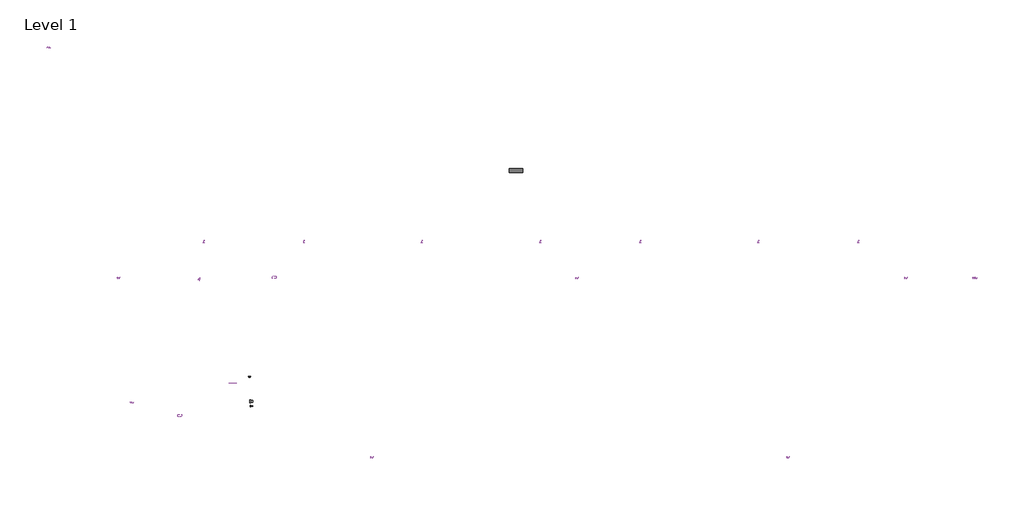
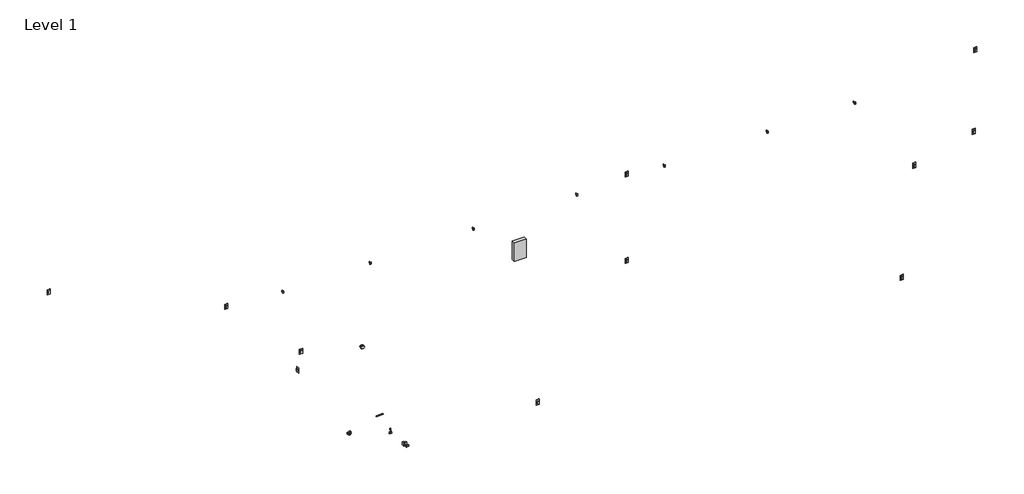
# One storey: 26 proxies.
# Revit data of these elements (continued)
# Type "Intruder Security Alarm Sounder : Standard" (continued)
#   Classification.MasterFormat.Number = "28 30 00"
#   Classification.OmniClass.23.Number = "23-29 11 23 15"
#   Classification.OmniClass.23.Description = "Intrusion Detection Microwave Alarms"
#   Classification.UniFormat.II.Number = "D7050"
#   COBie.Type.CreatedBy = "info@mma.ie"
#   COBie.Type.CreatedOn = "2017-07-26T09:25:07"
#   COBie.Type.Name = "Intruder Security Alarm Sounder"
#   COBie.Type.Category = "23-29 11 23 15 : Intrusion Detection Microwave Alarms"
#   COBie.Type.Description = "Intruder Security Alarm Sounder_Intruder Security Alarm Sounder"
#   COBie.Type.AssetType = "Fixed"
#   COBie.Type.Manufacturer = ""
#   COBie.Type.ModelNumber = ""
#   Standard = ""
#   SounderType = ""
#   SounderCutOffTimeMaximum = ""
#   PowerSupply = ""
#   Mounting = ""
#   Keynote = "28 01 30.51.A"
#   IntegralBeacon = ""
#   IngressProtectionStandard = ""
#   I.A. Audio Level = "75dB"
#   DirectionalOutputAt1MMinimum = ""
#   COBie.Type.ReplacementCost = 0
#   UsageCurrent = 0
#   SounderRadius = 75 mm
#   SounderDepth = 50 mm
#   PlanSymbolOffset [instance default] = 250 mm
#   PlanSymbolAlignment [instance default] = 0 mm
#   PhaseAngle = 0.00°
#   NominalVoltage = 0
#   NominalLength = 150 mm
#   NominalHeight = 80 mm
#   NominalFrequencyRange = 0
#   NominalCurrent = 0
#   I.A. Diameter = 150 mm
#   I.A. Depth = 50 mm
#   BaseLevelOffset = 0 mm
#   BackingCaseDepth = 30 mm
#   COBie.Type = yes
#   PlanSymbolVisibility [instance default] = yes
#   PlanObjectVisibility [instance default] = yes
#   NumberOfPoles = 0
#   HasProtectiveEarth = yes
#   URL = ""
#   Type Comments = ""
#   Model = ""
#   Manufacturer = ""
#   Description = (empty or 0)
#   Default Elevation = 0
#   Assembly Code = ""
# Type "Wall Mounted Passive Infrared Detector : Standard"
#   Type Mark = "Wall Mounted Passive Infrared Detector"
#   Classification.OmniClass.21.Number = "21-04 70 70 10"
#   Classification.OmniClass.21.Description = "Electronic Detention Monitoring and Control"
#   Classification.UniFormat.II.Description = "Intruction Detection"
#   Classification.OmniClass.23.Number = "23-29 11 21"
#   Classification.OmniClass.23.Description = "Security Sensors"
#   Classification.UniFormat.II.Number = "D7010.50"
#   COBie.Type.CreatedBy = "info@mma.ie"
#   COBie.Type.CreatedOn = "2017-07-26T09:12:44"
#   COBie.Type.Name = "Wall Mounted Passive Infrared Detector"
#   COBie.Type.Category = "23-29 11 21 : Security Sensors"
#   COBie.Type.Description = "Wall Mounted Passive Infrared Detector_Standard"
#   COBie.Type.AssetType = "Movable"
#   COBie.Type.Manufacturer = ""
#   COBie.Type.ModelNumber = ""
#   COBie.Type.ModelReference = ""
#   COBie.Type.Color = "White"
#   Units = "Volts"
#   Label = "PIR"
#   Keynote = "28 16 19.A"
#   COBie.Type.ReplacementCost = 0
#   Width 1 = 128 mm
#   Sensor Voltage = 230 V
#   PIR_Width = 64 mm
#   PIR_Depth = 53 mm
#   PIR Height = 117 mm
#   Length 1 = 234 mm
#   Height 1 = 3.312 mm
#   Default Elevation = 1200 mm
#   Sensor Width = 64 mm
#   Sensor Length = 117 mm
#   Sensor Height = 53 mm
#   Apparent Load = 0 VA
#   COBie.Type = yes
#   Sensor Number of Poles = 1
#   Sensor Material = none
#   Load Classification = Other
#   Cover Material = none
#   URL = ""
#   Model = ""
#   Manufacturer = ""
# Element 1 (IfcBuildingElementProxy, "Access Card Reader : Standard")
#   Comments = "2"
#   Mark = "1"
#   COBie.CreatedBy = "info@mma.ie"
#   COBie.CreatedOn = "2017-07-26T09:12:43"
#   COBie.Component.Name = "Access Card Reader-1"
#   COBie.Component.Space = "128"
#   COBie.Component.Description = "Access Card Reader: Standard"
#   Notes = "n/a"
#   Color = "Grey"
#   Voltage = 12 V
#   Power = 2.8 W
#   COBie = yes
#   Image = none
#   Phase Created = New Construction
# Element 2 (IfcBuildingElementProxy, "Access Card Reader : Standard")
#   Comments = "1"
#   Mark = "2"
#   COBie.CreatedBy = "info@mma.ie"
#   COBie.CreatedOn = "2017-07-26T09:12:43"
#   COBie.Component.Name = "Access Card Reader-2"
#   COBie.Component.Space = "217"
#   COBie.Component.Description = "Access Card Reader: Standard"
#   Notes = "n/a"
#   Color = "Grey"
#   Voltage = 12 V
#   Power = 2.8 W
#   COBie = yes
#   Phase Created = New Construction
# Element 3 (IfcBuildingElementProxy, "Access Card Reader : Standard")
#   Comments = "2"
#   Mark = "3"
#   COBie.CreatedBy = "info@mma.ie"
#   COBie.CreatedOn = "2017-07-26T09:12:43"
#   COBie.Component.Name = "Access Card Reader-3"
#   COBie.Component.Space = "217"
#   COBie.Component.Description = "Access Card Reader: Standard"
#   Notes = "n/a"
#   Color = "Grey"
#   Voltage = 12 V
#   Power = 2.8 W
#   COBie = yes
#   Phase Created = New Construction
# Element 4 (IfcBuildingElementProxy, "Access Card Reader : Standard")
#   Comments = "3"
#   Mark = "4"
#   COBie.CreatedBy = "info@mma.ie"
#   COBie.CreatedOn = "2017-07-26T09:12:43"
#   COBie.Component.Name = "Access Card Reader-4"
#   COBie.Component.Space = "217"
#   COBie.Component.Description = "Access Card Reader: Standard"
#   Notes = "n/a"
#   Color = "Grey"
#   Voltage = 12 V
#   Power = 2.8 W
#   COBie = yes
#   Phase Created = New Construction
# Element 5 (IfcBuildingElementProxy, "Access Card Reader : Standard")
#   Comments = "4"
#   Mark = "5"
#   COBie.CreatedBy = "info@mma.ie"
#   COBie.CreatedOn = "2017-07-26T09:12:43"
#   COBie.Component.Name = "Access Card Reader-5"
#   COBie.Component.Space = "217"
#   COBie.Component.Description = "Access Card Reader: Standard"
#   Notes = "n/a"
#   Color = "Grey"
#   Voltage = 12 V
#   Power = 2.8 W
#   COBie = yes
#   Phase Created = New Construction
# Element 6 (IfcBuildingElementProxy, "Access Card Reader : Standard")
#   Comments = "5"
#   Mark = "6"
#   COBie.CreatedBy = "info@mma.ie"
#   COBie.CreatedOn = "2017-07-26T09:12:43"
#   COBie.Component.Name = "Access Card Reader-6"
#   COBie.Component.Space = "217"
#   COBie.Component.Description = "Access Card Reader: Standard"
#   Notes = "n/a"
#   Color = "Grey"
#   Voltage = 12 V
#   Power = 2.8 W
#   COBie = yes
#   Phase Created = New Construction
# Element 7 (IfcBuildingElementProxy, "Access Card Reader : Standard")
#   Comments = "6"
#   Mark = "7"
#   COBie.CreatedBy = "info@mma.ie"
#   COBie.CreatedOn = "2017-07-26T09:12:43"
#   COBie.Component.Name = "Access Card Reader-7"
#   COBie.Component.Space = "217"
#   COBie.Component.Description = "Access Card Reader: Standard"
#   Notes = "n/a"
#   Color = "Grey"
#   Voltage = 12 V
#   Power = 2.8 W
#   COBie = yes
#   Phase Created = New Construction
# Element 8 (IfcBuildingElementProxy, "Access Card Reader : Standard")
#   Comments = "7"
#   Mark = "8"
#   COBie.CreatedBy = "info@mma.ie"
#   COBie.CreatedOn = "2017-07-26T09:12:43"
#   COBie.Component.Name = "Access Card Reader-8"
#   COBie.Component.Space = "217"
#   COBie.Component.Description = "Access Card Reader: Standard"
#   Notes = "n/a"
#   Color = "Grey"
#   Voltage = 12 V
#   Power = 2.8 W
#   COBie = yes
#   Phase Created = New Construction
# Element 9 (IfcBuildingElementProxy, "Bell : Standard")
#   Comments = "1"
#   Mark = "1"
#   COBie.CreatedBy = "info@mma.ie"
#   COBie.CreatedOn = "2017-07-26T09:12:43"
#   COBie.Component.Name = "Bell-1"
#   COBie.Component.Space = "128"
#   COBie.Component.Description = "Bell: Standard"
#   Notes = "n/a"
#   Color = "Silver"
#   Voltage = 12 V
#   Power = 2.8 W
#   COBie = yes
#   Phase Created = New Construction
# Element 10 (IfcBuildingElementProxy, "Door Lock Magnetic : Standard")
#   Comments = "14"
#   Mark = "1"
#   COBie.CreatedBy = "info@mma.ie"
#   COBie.CreatedOn = "2017-07-26T09:12:43"
#   COBie.Component.Name = "Door Lock Magnetic-1"
#   COBie.Component.Space = "123"
#   COBie.Component.Description = "Door Lock Magnetic: Standard"
#   Notes = "n/a"
#   Color = "Stainless Steel"
#   Voltage = 12 V
#   Power = 2.8 W
#   COBie = yes
#   Phase Created = New Construction
# Element 11 (IfcBuildingElementProxy, "Keypad : Standard")
#   Mark = "1"
#   COBie.CreatedBy = "info@mma.ie"
#   COBie.CreatedOn = "2017-07-26T09:12:43"
#   COBie.Component.Name = "Keypad-1"
#   COBie.Component.Space = "123"
#   COBie.Component.Description = "Keypad: Standard"
#   Notes = "n/a"
#   Color = "Stainless Steel"
#   Voltage = 12 V
#   Power = 3 W
#   COBie = yes
#   Phase Created = New Construction
# Element 12 (IfcBuildingElementProxy, "Release Button : Standard")
#   Comments = "5"
#   Mark = "1"
#   COBie.CreatedBy = "info@mma.ie"
#   COBie.CreatedOn = "2017-07-26T09:12:43"
#   COBie.Component.Name = "Release Button-1"
#   COBie.Component.Space = "123"
#   COBie.Component.Description = "Release Button: Standard"
#   Notes = "n/a"
#   Color = "Stainless Steel"
#   Voltage = 24 V
#   Power = 2.8 W
#   COBie = yes
#   Phase Created = New Construction
# Element 13 (IfcBuildingElementProxy, "Security Panel : 225 A")
#   Panel Name = "SP1"
#   Mark = "1"
#   COBie.CreatedBy = "info@mma.ie"
#   COBie.CreatedOn = "2017-07-26T09:12:43"
#   COBie.Component.Name = "Security Panel-1"
#   COBie.Component.Space = "107"
#   COBie.Component.Description = "Security Panel: 225 A"
#   Notes = "n/a"
#   Color = "Black"
#   built-in parameter 1140081 = "Recessed"
#   built-in parameter 1140083 = "Type 1"
#   Voltage = 208 V
#   built-in parameter 1140082 = 100 (stored number, unit not read)
#   Height = 812.8 mm
#   COBie = yes
#   built-in parameter 1140079 = 18
#   built-in parameter 1140064 = 120/208 Wye
#   Phase Created = New Construction
# Element 14 (IfcBuildingElementProxy, "Intruder Security Alarm Sounder : Standard")
#   Mark = "1"
#   COBie.CreatedBy = "info@mma.ie"
#   COBie.CreatedOn = "2017-07-26T09:12:43"
#   COBie.Component.Name = "Intruder Security Alarm Sounder-1"
#   COBie.Component.Space = "117"
#   COBie.Component.Description = "Intruder Security Alarm Sounder: Intruder Security Alarm Sounder"
#   Notes = "n/a"
#   Color = "Red"
#   Voltage = 24 V
#   Power = 0.6 W
#   PlanSymbolOffset = 250 mm
#   PlanSymbolAlignment = 0 mm
#   COBie = yes
#   PlanSymbolVisibility = yes
#   PlanObjectVisibility = yes
#   Phase Created = New Construction
#   Materials on its faces: "nbl_ConceptWhite"
# Element 15 (IfcBuildingElementProxy, "Intruder Security Alarm Sounder : Standard")
#   Mark = "2"
#   COBie.CreatedBy = "info@mma.ie"
#   COBie.CreatedOn = "2017-07-26T09:12:43"
#   COBie.Component.Name = "Intruder Security Alarm Sounder-2"
#   COBie.Component.Space = "128"
#   COBie.Component.Description = "Intruder Security Alarm Sounder: Intruder Security Alarm Sounder"
#   Notes = "n/a"
#   Color = "Red"
#   Voltage = 24 V
#   Power = 0.6 W
#   PlanSymbolOffset = 250 mm
#   PlanSymbolAlignment = 0 mm
#   COBie = yes
#   PlanSymbolVisibility = yes
#   PlanObjectVisibility = yes
#   Phase Created = New Construction
#   Materials on its faces: "nbl_ConceptWhite"
# Element 16 (IfcBuildingElementProxy, "Wall Mounted Passive Infrared Detector : Standard")
#   Comments = "6"
#   Mark = "1"
#   COBie.CreatedBy = "info@mma.ie"
#   COBie.CreatedOn = "2017-07-26T09:12:43"
#   COBie.Component.Name = "Wall Mounted Passive Infrared Detector-1"
#   COBie.Component.Space = "117"
#   COBie.Component.Description = "Wall Mounted Passive Infrared Detector: Standard"
#   Notes = "n/a"
#   Color = "White"
#   Voltage = 12 V
#   Power = 0.15 W
#   COBie = yes
#   Phase Created = New Construction
# Element 17 (IfcBuildingElementProxy, "Wall Mounted Passive Infrared Detector : Standard")
#   Comments = "8"
#   Mark = "2"
#   COBie.CreatedBy = "info@mma.ie"
#   COBie.CreatedOn = "2017-07-26T09:12:43"
#   COBie.Component.Name = "Wall Mounted Passive Infrared Detector-2"
#   COBie.Component.Space = "101"
#   COBie.Component.Description = "Wall Mounted Passive Infrared Detector: Standard"
#   Notes = "n/a"
#   Color = "White"
#   Voltage = 12 V
#   Power = 0.15 W
#   COBie = yes
#   Phase Created = New Construction
# Element 18 (IfcBuildingElementProxy, "Wall Mounted Passive Infrared Detector : Standard")
#   Comments = "9"
#   Mark = "3"
#   COBie.CreatedBy = "info@mma.ie"
#   COBie.CreatedOn = "2017-07-26T09:12:43"
#   COBie.Component.Name = "Wall Mounted Passive Infrared Detector-3"
#   COBie.Component.Space = "118"
#   COBie.Component.Description = "Wall Mounted Passive Infrared Detector: Standard"
#   Notes = "n/a"
#   Color = "White"
#   Voltage = 12 V
#   Power = 0.15 W
#   COBie = yes
#   Phase Created = New Construction
# Element 19 (IfcBuildingElementProxy, "Wall Mounted Passive Infrared Detector : Standard")
#   Comments = "8"
#   Mark = "4"
#   COBie.CreatedBy = "info@mma.ie"
#   COBie.CreatedOn = "2017-07-26T09:12:43"
#   COBie.Component.Name = "Wall Mounted Passive Infrared Detector-4"
#   COBie.Component.Space = "217"
#   COBie.Component.Description = "Wall Mounted Passive Infrared Detector: Standard"
#   Notes = "n/a"
#   Color = "White"
#   Voltage = 12 V
#   Power = 0.15 W
#   COBie = yes
#   Phase Created = New Construction
# Element 20 (IfcBuildingElementProxy, "Wall Mounted Passive Infrared Detector : Standard")
#   Comments = "10"
#   Mark = "6"
#   COBie.CreatedBy = "info@mma.ie"
#   COBie.CreatedOn = "2017-07-26T09:12:43"
#   COBie.Component.Name = "Wall Mounted Passive Infrared Detector-6"
#   COBie.Component.Space = "217"
#   COBie.Component.Description = "Wall Mounted Passive Infrared Detector: Standard"
#   Notes = "n/a"
#   Color = "White"
#   Voltage = 12 V
#   Power = 0.15 W
#   COBie = yes
#   Phase Created = New Construction
# Element 21 (IfcBuildingElementProxy, "Wall Mounted Passive Infrared Detector : Standard")
#   Comments = "12"
#   Mark = "7"
#   COBie.CreatedBy = "info@mma.ie"
#   COBie.CreatedOn = "2017-07-26T09:12:43"
#   COBie.Component.Name = "Wall Mounted Passive Infrared Detector-7"
#   COBie.Component.Space = "116"
#   COBie.Component.Description = "Wall Mounted Passive Infrared Detector: Standard"
#   Notes = "n/a"
#   Color = "White"
#   Voltage = 12 V
#   Power = 0.15 W
#   COBie = yes
#   Phase Created = New Construction
# Element 22 (IfcBuildingElementProxy, "Wall Mounted Passive Infrared Detector : Standard")
#   Comments = "11"
#   Mark = "8"
#   COBie.CreatedBy = "info@mma.ie"
#   COBie.CreatedOn = "2017-07-26T09:12:43"
#   COBie.Component.Name = "Wall Mounted Passive Infrared Detector-8"
#   COBie.Component.Space = "219"
#   COBie.Component.Description = "Wall Mounted Passive Infrared Detector: Standard"
#   Notes = "n/a"
#   Color = "White"
#   Voltage = 12 V
#   Power = 0.15 W
#   COBie = yes
#   Phase Created = New Construction
# Element 23 (IfcBuildingElementProxy, "Wall Mounted Passive Infrared Detector : Standard")
#   Comments = "12"
#   Mark = "9"
#   COBie.CreatedBy = "info@mma.ie"
#   COBie.CreatedOn = "2017-07-26T09:12:43"
#   COBie.Component.Name = "Wall Mounted Passive Infrared Detector-9"
#   COBie.Component.Space = "218"
#   COBie.Component.Description = "Wall Mounted Passive Infrared Detector: Standard"
#   Notes = "n/a"
#   Color = "White"
#   Voltage = 12 V
#   Power = 0.15 W
#   COBie = yes
#   Phase Created = New Construction
# Element 24 (IfcBuildingElementProxy, "Wall Mounted Passive Infrared Detector : Standard")
#   Comments = "16"
#   Mark = "10"
#   COBie.CreatedBy = "info@mma.ie"
#   COBie.CreatedOn = "2017-07-26T09:12:43"
#   COBie.Component.Name = "Wall Mounted Passive Infrared Detector-10"
#   COBie.Component.Space = "117"
#   COBie.Component.Description = "Wall Mounted Passive Infrared Detector: Standard"
#   Notes = "n/a"
#   Color = "White"
#   Voltage = 12 V
#   Power = 0.15 W
#   COBie = yes
#   Phase Created = New Construction
# Element 25 (IfcBuildingElementProxy, "Wall Mounted Passive Infrared Detector : Standard")
#   Comments = "17"
#   Mark = "11"
#   COBie.CreatedBy = "info@mma.ie"
#   COBie.CreatedOn = "2017-07-26T09:12:43"
#   COBie.Component.Name = "Wall Mounted Passive Infrared Detector-11"
#   COBie.Component.Space = "123"
#   COBie.Component.Description = "Wall Mounted Passive Infrared Detector: Standard"
#   Notes = "n/a"
#   Color = "White"
#   Voltage = 12 V
#   Power = 0.15 W
#   COBie = yes
#   Phase Created = New Construction
# Element 26 (IfcBuildingElementProxy, "Wall Mounted Passive Infrared Detector : Standard")
#   Comments = "9"
#   Mark = "12"
#   COBie.CreatedBy = "info@mma.ie"
#   COBie.CreatedOn = "2017-07-26T09:12:43"
#   COBie.Component.Name = "Wall Mounted Passive Infrared Detector-12"
#   COBie.Component.Space = "121"
#   COBie.Component.Description = "Wall Mounted Passive Infrared Detector: Standard"
#   Notes = "n/a"
#   Color = "White"
#   Voltage = 12 V
#   Power = 0.15 W
#   COBie = yes
#   Phase Created = New Construction
# Materials
#   "nbl_ConceptWhite": class "Generic", colour RGB 255 255 255, transparency 0, Cost = 0
# Space at (25106.444, 9340) mm, phase "New Construction", upper level "Level 2", upper offset -200 mm, lower offset 0 mm
#   Number = "111"
#   Name = "Storage"
#   Classification.Space.Number = "13-63 13 11"
#   Classification.Space.Description = "Storage Room"
#   COBie.CreatedBy = "info@mma.ie"
#   COBie.CreatedOn = "2017-07-26T09:12:43"
#   COBie.Space.Name = "111"
#   COBie.Space.Category = "13-63 13 11 : Storage Room"
#   COBie.Space.Description = "Storage"
#   Actual Lighting Load per area = 0
#   Actual Power Load per area = 0
#   Sensible Heat Gain per person = 0
#   Specified Lighting Load = 73041.7 (stored number, unit not read)
#   Specified Power Load = 94954.2 (stored number, unit not read)
#   Latent Heat Gain per person = 0
#   Total Heat Gain per person = 0
#   Area per Person = 0
#   Number of People = 22.0647 (stored number, unit not read)
#   COBie.Space.UsableHeight = 3600 mm
#   COBie.Space.GrossArea = 5.21302 m²
#   COBie.Space.NetArea = 0 m²
#   Lighting Load Units = 0
#   Power Load Units = 0
#   Return Airflow = 0
#   Occupancy Unit = -1
#   Condition Type = 2
#   COBie = yes
#   Construction Type = none
# Space at (-3466.111, 10795.59) mm, phase "New Construction", upper level "Level 2", upper offset 0 mm, lower offset 0 mm
#   Number = "001"
#   Name = "Exercise Terrace"
#   Classification.Space.Number = "13-33 11 15 41"
#   Classification.Space.Description = "Exercise Space"
#   COBie.CreatedBy = "info@mma.ie"
#   COBie.CreatedOn = "2017-07-26T09:12:43"
#   COBie.Space.Name = "001"
#   COBie.Space.Category = "13-33 11 15 41 : Exercise Space"
#   COBie.Space.Description = "Exercise Terrace"
#   Actual Lighting Load per area = 0
#   Actual Power Load per area = 0
#   Sensible Heat Gain per person = 0
#   Specified Lighting Load = 5865.96 (stored number, unit not read)
#   Specified Power Load = 7625.74 (stored number, unit not read)
#   Latent Heat Gain per person = 0
#   Total Heat Gain per person = 0
#   Area per Person = 0
#   Number of People = 1.77201 (stored number, unit not read)
#   COBie.Space.UsableHeight = 3800 mm
#   COBie.Space.GrossArea = 46.8469 m²
#   COBie.Space.NetArea = 0 m²
#   Lighting Load Units = 0
#   Power Load Units = 0
#   Return Airflow = 0
#   Occupancy Unit = -1
#   Condition Type = 2
#   COBie = yes
#   Construction Type = none
# Space at (6778.21, 4377.979) mm, phase "New Construction", upper level "Level 2", upper offset -200 mm, lower offset 0 mm
#   Number = "123"
#   Name = "Entry"
#   Classification.Space.Number = "13-25"
#   Classification.Space.Description = "Circulation Spaces"
#   COBie.CreatedBy = "info@mma.ie"
#   COBie.CreatedOn = "2017-07-26T09:12:43"
#   COBie.Space.Name = "123"
#   COBie.Space.Category = "13-25 : Circulation Spaces"
#   COBie.Space.Description = "Entry"
#   Actual Lighting Load per area = 0
#   Actual Power Load per area = 0
#   Sensible Heat Gain per person = 0
#   Specified Lighting Load = 1051.01 (stored number, unit not read)
#   Specified Power Load = 1366.31 (stored number, unit not read)
#   Latent Heat Gain per person = 0
#   Total Heat Gain per person = 0
#   Area per Person = 0
#   Number of People = 0.317492 (stored number, unit not read)
#   COBie.Space.UsableHeight = 3600 mm
#   COBie.Space.GrossArea = 7.40986 m²
#   COBie.Space.NetArea = 0 m²
#   Lighting Load Units = 0
#   Power Load Units = 0
#   Return Airflow = 0
#   Occupancy Unit = -1
#   Condition Type = 2
#   COBie = yes
#   Construction Type = none
# Space at (6131.224, -2983.196) mm, phase "New Construction", upper level "Level 1", upper offset 2000 mm, lower offset 0 mm
#   Number = "128"
#   Name = "External Space Level 1"
#   Classification.Space.Number = "13-25 17"
#   Classification.Space.Description = "External Circulation Spaces"
#   COBie.CreatedBy = "info@mma.ie"
#   COBie.CreatedOn = "2017-07-26T09:12:43"
#   COBie.Space.Name = "128"
#   COBie.Space.Category = "13-25 17 : External Circulation Spaces"
#   COBie.Space.Description = "External Circulation Spaces"
#   Actual Lighting Load per area = 0
#   Actual Power Load per area = 0
#   Sensible Heat Gain per person = 0
#   Specified Lighting Load = 80587.6 (stored number, unit not read)
#   Specified Power Load = 104763.9 (stored number, unit not read)
#   Latent Heat Gain per person = 0
#   Total Heat Gain per person = 0
#   Area per Person = 0
#   Number of People = 24.3442 (stored number, unit not read)
#   COBie.Space.UsableHeight = 2000 mm
#   COBie.Space.GrossArea = 695.172 m²
#   COBie.Space.NetArea = 0 m²
#   Lighting Load Units = 0
#   Power Load Units = 0
#   Return Airflow = 0
#   Occupancy Unit = -1
#   Condition Type = 2
#   COBie = yes
#   Construction Type = none
# Space at (30095.163, 9340) mm, phase "New Construction", upper level "Level 2", upper offset -200 mm, lower offset 0 mm
#   Number = "114"
#   Name = "Pantry"
#   Classification.Space.Number = "13-57 13 13"
#   Classification.Space.Description = "Kitchen Space"
#   COBie.CreatedBy = "info@mma.ie"
#   COBie.CreatedOn = "2017-07-26T09:12:43"
#   COBie.Space.Name = "114"
#   COBie.Space.Category = "13-57 13 13 : Kitchen Space"
#   COBie.Space.Description = "Pantry"
#   Actual Lighting Load per area = 0
#   Actual Power Load per area = 0
#   Sensible Heat Gain per person = 0
#   Specified Lighting Load = 0
#   Specified Power Load = 0
#   Latent Heat Gain per person = 0
#   Total Heat Gain per person = 0
#   Area per Person = 0
#   Number of People = 0.339922 (stored number, unit not read)
#   COBie.Space.UsableHeight = 3600 mm
#   COBie.Space.GrossArea = 9.71206 m²
#   COBie.Space.NetArea = 0 m²
#   Lighting Load Units = 0
#   Power Load Units = 0
#   Return Airflow = 0
#   Occupancy Unit = -1
#   Condition Type = 2
#   COBie = yes
#   Construction Type = none
# Space at (13314.806, 9198.95) mm, phase "New Construction", upper level "Level 2", upper offset -200 mm, lower offset 0 mm
#   Number = "104"
#   Name = "Storage"
#   Classification.Space.Number = "13-63 13 11"
#   Classification.Space.Description = "Storage Room"
#   COBie.CreatedBy = "info@mma.ie"
#   COBie.CreatedOn = "2017-07-26T09:12:43"
#   COBie.Space.Name = "104"
#   COBie.Space.Category = "13-63 13 11 : Storage Room"
#   COBie.Space.Description = "Storage"
#   Actual Lighting Load per area = 0
#   Actual Power Load per area = 0
#   Sensible Heat Gain per person = 0
#   Specified Lighting Load = 0
#   Specified Power Load = 0
#   Latent Heat Gain per person = 0
#   Total Heat Gain per person = 0
#   Area per Person = 0
#   Number of People = 0.36309 (stored number, unit not read)
#   COBie.Space.UsableHeight = 3600 mm
#   COBie.Space.GrossArea = 10.374 m²
#   COBie.Space.NetArea = 0 m²
#   Lighting Load Units = 0
#   Power Load Units = 0
#   Return Airflow = 0
#   Occupancy Unit = -1
#   Condition Type = 2
#   COBie = yes
#   Construction Type = none
# Space at (17230.963, 11648.082) mm, phase "New Construction", upper level "Level 2", upper offset -200 mm, lower offset 0 mm
#   Number = "107"
#   Name = "Closet"
#   Classification.Space.Number = "13-63 13 13"
#   Classification.Space.Description = "Closet"
#   COBie.CreatedBy = "info@mma.ie"
#   COBie.CreatedOn = "2017-07-26T09:12:43"
#   COBie.Space.Name = "107"
#   COBie.Space.Category = "13-63 13 13 : Closet"
#   COBie.Space.Description = "Closet"
#   Actual Lighting Load per area = 0
#   Actual Power Load per area = 0
#   Sensible Heat Gain per person = 0
#   Specified Lighting Load = 0
#   Specified Power Load = 0
#   Latent Heat Gain per person = 0
#   Total Heat Gain per person = 0
#   Area per Person = 0
#   Number of People = 0.0932222 (stored number, unit not read)
#   COBie.Space.UsableHeight = 3600 mm
#   COBie.Space.GrossArea = 2.66349 m²
#   COBie.Space.NetArea = 0 m²
#   Lighting Load Units = 0
#   Power Load Units = 0
#   Return Airflow = 0
#   Occupancy Unit = -1
#   Condition Type = 2
#   COBie = yes
#   Construction Type = none
# Space at (17230.963, 9449.188) mm, phase "New Construction", upper level "Level 2", upper offset -200 mm, lower offset 0 mm
#   Number = "109"
#   Name = "Elec/Tel"
#   Classification.Space.Number = "13-23 19 27"
#   Classification.Space.Description = "Electrical Room"
#   COBie.CreatedBy = "info@mma.ie"
#   COBie.CreatedOn = "2017-07-26T09:12:43"
#   COBie.Space.Name = "109"
#   COBie.Space.Category = "13-23 19 27 : Electrical Room"
#   COBie.Space.Description = "Elec/Tel"
#   Actual Lighting Load per area = 0
#   Actual Power Load per area = 0
#   Sensible Heat Gain per person = 0
#   Specified Lighting Load = 0
#   Specified Power Load = 0
#   Latent Heat Gain per person = 0
#   Total Heat Gain per person = 0
#   Area per Person = 0
#   Number of People = 0.141204 (stored number, unit not read)
#   COBie.Space.UsableHeight = 3600 mm
#   COBie.Space.GrossArea = 4.03441 m²
#   COBie.Space.NetArea = 0 m²
#   Lighting Load Units = 0
#   Power Load Units = 0
#   Return Airflow = 0
#   Occupancy Unit = -1
#   Condition Type = 2
#   COBie = yes
#   Construction Type = none
# Space at (20994.025, 9449.188) mm, phase "New Construction", upper level "Level 2", upper offset -200 mm, lower offset 0 mm
#   Number = "110"
#   Name = "Laundry"
#   Classification.Space.Number = "13-65 17"
#   Classification.Space.Description = "Laundry Room"
#   COBie.CreatedBy = "info@mma.ie"
#   COBie.CreatedOn = "2017-07-26T09:12:43"
#   COBie.Space.Name = "110"
#   COBie.Space.Category = "13-65 17 : Laundry Room"
#   COBie.Space.Description = "Laundry"
#   Actual Lighting Load per area = 0
#   Actual Power Load per area = 0
#   Sensible Heat Gain per person = 0
#   Specified Lighting Load = 0
#   Specified Power Load = 0
#   Latent Heat Gain per person = 0
#   Total Heat Gain per person = 0
#   Area per Person = 0
#   Number of People = 0.437432 (stored number, unit not read)
#   COBie.Space.UsableHeight = 3600 mm
#   COBie.Space.GrossArea = 12.4981 m²
#   COBie.Space.NetArea = 0 m²
#   Lighting Load Units = 0
#   Power Load Units = 0
#   Return Airflow = 0
#   Occupancy Unit = -1
#   Condition Type = 2
#   COBie = yes
#   Construction Type = none
# Space at (9483.263, 9198.95) mm, phase "New Construction", upper level "Level 2", upper offset -200 mm, lower offset 0 mm
#   Number = "103"
#   Name = "Toilet"
#   Classification.Space.Number = "13-65 13 13"
#   Classification.Space.Description = "Toilet Space"
#   COBie.CreatedBy = "info@mma.ie"
#   COBie.CreatedOn = "2017-07-26T09:12:43"
#   COBie.Space.Name = "103"
#   COBie.Space.Category = "13-65 13 13 : Toilet Space"
#   COBie.Space.Description = "Toilet"
#   Actual Lighting Load per area = 0
#   Actual Power Load per area = 0
#   Sensible Heat Gain per person = 0
#   Specified Lighting Load = 0
#   Specified Power Load = 0
#   Latent Heat Gain per person = 0
#   Total Heat Gain per person = 0
#   Area per Person = 0
#   Number of People = 0.146893 (stored number, unit not read)
#   COBie.Space.UsableHeight = 3600 mm
#   COBie.Space.GrossArea = 4.19694 m²
#   COBie.Space.NetArea = 0 m²
#   Lighting Load Units = 0
#   Power Load Units = 0
#   Return Airflow = 0
#   Occupancy Unit = -1
#   Condition Type = 2
#   COBie = yes
#   Construction Type = none
# Space at (7140.7, 9198.95) mm, phase "New Construction", upper level "Level 2", upper offset -200 mm, lower offset 0 mm
#   Number = "102"
#   Name = "Toilet"
#   Classification.Space.Number = "13-65 13 13"
#   Classification.Space.Description = "Toilet Space"
#   COBie.CreatedBy = "info@mma.ie"
#   COBie.CreatedOn = "2017-07-26T09:12:43"
#   COBie.Space.Name = "102"
#   COBie.Space.Category = "13-65 13 13 : Toilet Space"
#   COBie.Space.Description = "Toilet"
#   Actual Lighting Load per area = 0
#   Actual Power Load per area = 0
#   Sensible Heat Gain per person = 0
#   Specified Lighting Load = 0
#   Specified Power Load = 0
#   Latent Heat Gain per person = 0
#   Total Heat Gain per person = 0
#   Area per Person = 0
#   Number of People = 0.146751 (stored number, unit not read)
#   COBie.Space.UsableHeight = 3600 mm
#   COBie.Space.GrossArea = 4.19289 m²
#   COBie.Space.NetArea = 0 m²
#   Lighting Load Units = 0
#   Power Load Units = 0
#   Return Airflow = 0
#   Occupancy Unit = -1
#   Condition Type = 2
#   COBie = yes
#   Construction Type = none
# Space at (17230.963, 13855.144) mm, phase "New Construction", upper level "Level 2", upper offset -200 mm, lower offset 0 mm
#   Number = "106"
#   Name = "Bath"
#   Classification.Space.Number = "13-65 13"
#   Classification.Space.Description = "Bathroom"
#   COBie.CreatedBy = "info@mma.ie"
#   COBie.CreatedOn = "2017-07-26T09:12:43"
#   COBie.Space.Name = "106"
#   COBie.Space.Category = "13-65 13  : Bathroom"
#   COBie.Space.Description = "Bath"
#   Actual Lighting Load per area = 0
#   Actual Power Load per area = 0
#   Sensible Heat Gain per person = 0
#   Specified Lighting Load = 0
#   Specified Power Load = 0
#   Latent Heat Gain per person = 0
#   Total Heat Gain per person = 0
#   Area per Person = 0
#   Number of People = 0.141421 (stored number, unit not read)
#   COBie.Space.UsableHeight = 3600 mm
#   COBie.Space.GrossArea = 4.0406 m²
#   COBie.Space.NetArea = 0 m²
#   Lighting Load Units = 0
#   Power Load Units = 0
#   Return Airflow = 0
#   Occupancy Unit = -1
#   Condition Type = 2
#   COBie = yes
#   Construction Type = none
# Space at (19950.244, 12967.938) mm, phase "New Construction", upper level "Level 2", upper offset -200 mm, lower offset 0 mm
#   Number = "108"
#   Name = "Break Room"
#   Classification.Space.Number = "13-57 17 13"
#   Classification.Space.Description = "Break Room"
#   COBie.CreatedBy = "info@mma.ie"
#   COBie.CreatedOn = "2017-07-26T09:12:43"
#   COBie.Space.Name = "108"
#   COBie.Space.Category = "13-57 17 13 : Break Room"
#   COBie.Space.Description = "Break Room"
#   Actual Lighting Load per area = 0
#   Actual Power Load per area = 0
#   Sensible Heat Gain per person = 0
#   Specified Lighting Load = 0
#   Specified Power Load = 0
#   Latent Heat Gain per person = 0
#   Total Heat Gain per person = 0
#   Area per Person = 0
#   Number of People = 0.538984 (stored number, unit not read)
#   COBie.Space.UsableHeight = 3600 mm
#   COBie.Space.GrossArea = 15.3995 m²
#   COBie.Space.NetArea = 0 m²
#   Lighting Load Units = 0
#   Power Load Units = 0
#   Return Airflow = 0
#   Occupancy Unit = -1
#   Condition Type = 2
#   COBie = yes
#   Construction Type = none
# Space at (30744.45, 12858.75) mm, phase "New Construction", upper level "Level 2", upper offset -200 mm, lower offset 0 mm
#   Number = "113"
#   Name = "Food Storage"
#   Classification.Space.Number = "13-63 13 11"
#   Classification.Space.Description = "Storage Room"
#   COBie.CreatedBy = "info@mma.ie"
#   COBie.CreatedOn = "2017-07-26T09:12:43"
#   COBie.Space.Name = "113"
#   COBie.Space.Category = "13-63 13 11 : Storage Room"
#   COBie.Space.Description = "Food Storage"
#   Actual Lighting Load per area = 0
#   Actual Power Load per area = 0
#   Sensible Heat Gain per person = 0
#   Specified Lighting Load = 0
#   Specified Power Load = 0
#   Latent Heat Gain per person = 0
#   Total Heat Gain per person = 0
#   Area per Person = 0
#   Number of People = 0.465855 (stored number, unit not read)
#   COBie.Space.UsableHeight = 3600 mm
#   COBie.Space.GrossArea = 13.3101 m²
#   COBie.Space.NetArea = 0 m²
#   Lighting Load Units = 0
#   Power Load Units = 0
#   Return Airflow = 0
#   Occupancy Unit = -1
#   Condition Type = 2
#   COBie = yes
#   Construction Type = none
# Space at (33531.25, 14017.509) mm, phase "New Construction", upper level "Level 2", upper offset -200 mm, lower offset 0 mm
#   Number = "115"
#   Name = "Outdoor Storage"
#   Classification.Space.Number = "13-63 13 11"
#   Classification.Space.Description = "Storage Room"
#   COBie.CreatedBy = "info@mma.ie"
#   COBie.CreatedOn = "2017-07-26T09:12:43"
#   COBie.Space.Name = "115"
#   COBie.Space.Category = "13-63 13 11 : Storage Room"
#   COBie.Space.Description = "Outdoor Storage"
#   Actual Lighting Load per area = 0
#   Actual Power Load per area = 0
#   Sensible Heat Gain per person = 0
#   Specified Lighting Load = 0
#   Specified Power Load = 0
#   Latent Heat Gain per person = 0
#   Total Heat Gain per person = 0
#   Area per Person = 0
#   Number of People = 0.183416 (stored number, unit not read)
#   COBie.Space.UsableHeight = 3600 mm
#   COBie.Space.GrossArea = 5.24046 m²
#   COBie.Space.NetArea = 0 m²
#   Lighting Load Units = 0
#   Power Load Units = 0
#   Return Airflow = 0
#   Occupancy Unit = -1
#   Condition Type = 2
#   COBie = yes
#   Construction Type = none
# Space at (12216.125, 12750.2) mm, phase "New Construction", upper level "Level 2", upper offset -200 mm, lower offset 0 mm
#   Number = "105"
#   Name = "Mechanical Room"
#   Classification.Space.Number = "13-23 19"
#   Classification.Space.Description = "Utility Equipment Room"
#   COBie.CreatedBy = "info@mma.ie"
#   COBie.CreatedOn = "2017-07-26T09:12:43"
#   COBie.Space.Name = "105"
#   COBie.Space.Category = "13-23 19 : Utility Equipment Room"
#   COBie.Space.Description = "Mechanical Room"
#   Actual Lighting Load per area = 0
#   Actual Power Load per area = 0
#   Sensible Heat Gain per person = 0
#   Specified Lighting Load = 0
#   Specified Power Load = 0
#   Latent Heat Gain per person = 0
#   Total Heat Gain per person = 0
#   Area per Person = 0
#   Number of People = 1.28766 (stored number, unit not read)
#   COBie.Space.UsableHeight = 3600 mm
#   COBie.Space.GrossArea = 36.7902 m²
#   COBie.Space.NetArea = 0 m²
#   Lighting Load Units = 0
#   Power Load Units = 0
#   Return Airflow = 0
#   Occupancy Unit = -1
#   Condition Type = 2
#   COBie = yes
#   Construction Type = none
# Space at (4303.153, 2552.509) mm, phase "New Construction", upper level "Level 2", upper offset -200 mm, lower offset 0 mm
#   Number = "124"
#   Name = "Closet"
#   Classification.Space.Number = "13-63 13 13"
#   Classification.Space.Description = "Closet"
#   COBie.CreatedBy = "info@mma.ie"
#   COBie.CreatedOn = "2017-07-26T09:12:43"
#   COBie.Space.Name = "124"
#   COBie.Space.Category = "13-63 13 13 : Closet"
#   COBie.Space.Description = "Closet"
#   Actual Lighting Load per area = 0
#   Actual Power Load per area = 0
#   Sensible Heat Gain per person = 0
#   Specified Lighting Load = 0
#   Specified Power Load = 0
#   Latent Heat Gain per person = 0
#   Total Heat Gain per person = 0
#   Area per Person = 0
#   Number of People = 0.566835 (stored number, unit not read)
#   COBie.Space.UsableHeight = 3600 mm
#   COBie.Space.GrossArea = 1.97733 m²
#   COBie.Space.NetArea = 0 m²
#   Lighting Load Units = 0
#   Power Load Units = 0
#   Return Airflow = 0
#   Occupancy Unit = -1
#   Condition Type = 2
#   COBie = yes
#   Construction Type = none
# Space at (10643.48, 2189.733) mm, phase "New Construction", upper level "Level 2", upper offset -200 mm, lower offset 0 mm
#   Number = "121"
#   Name = "Living Room"
#   Classification.Space.Number = "13-65"
#   Classification.Space.Description = "Private Residential Spaces"
#   COBie.CreatedBy = "info@mma.ie"
#   COBie.CreatedOn = "2017-07-26T09:12:43"
#   COBie.Space.Name = "121"
#   COBie.Space.Category = "13-65 : Private Residential Spaces"
#   COBie.Space.Description = "Living Room"
#   Actual Lighting Load per area = 0
#   Actual Power Load per area = 0
#   Sensible Heat Gain per person = 0
#   Specified Lighting Load = 0
#   Specified Power Load = 0
#   Latent Heat Gain per person = 0
#   Total Heat Gain per person = 0
#   Area per Person = 0
#   Number of People = 4.33951 (stored number, unit not read)
#   COBie.Space.UsableHeight = 3600 mm
#   COBie.Space.GrossArea = 17.5909 m²
#   COBie.Space.NetArea = 0 m²
#   Lighting Load Units = 0
#   Power Load Units = 0
#   Return Airflow = 0
#   Occupancy Unit = -1
#   Condition Type = 2
#   COBie = yes
#   Construction Type = none
# Space at (19128.713, 7381.25) mm, phase "New Construction", upper level "Level 2", upper offset -200 mm, lower offset 0 mm
#   Number = "117"
#   Name = "Hall"
#   Classification.Space.Number = "13-25"
#   Classification.Space.Description = "Circulation Spaces"
#   COBie.CreatedBy = "info@mma.ie"
#   COBie.CreatedOn = "2017-07-26T09:12:43"
#   COBie.Space.Name = "117"
#   COBie.Space.Category = "13-25 : Circulation Spaces"
#   COBie.Space.Description = "Hall"
#   Actual Lighting Load per area = 0
#   Actual Power Load per area = 0
#   Sensible Heat Gain per person = 0
#   Specified Lighting Load = 0
#   Specified Power Load = 0
#   Latent Heat Gain per person = 0
#   Total Heat Gain per person = 0
#   Area per Person = 0
#   Number of People = 1.26052 (stored number, unit not read)
#   COBie.Space.UsableHeight = 3600 mm
#   COBie.Space.GrossArea = 36.0148 m²
#   COBie.Space.NetArea = 0 m²
#   Lighting Load Units = 0
#   Power Load Units = 0
#   Return Airflow = 0
#   Occupancy Unit = -1
#   Condition Type = 2
#   COBie = yes
#   Construction Type = none
# Space at (9068.849, 5264.733) mm, phase "New Construction", upper level "Level 2", upper offset -200 mm, lower offset 0 mm
#   Number = "122"
#   Name = "Closet"
#   Classification.Space.Number = "13-65 13 13"
#   Classification.Space.Description = "Closet"
#   COBie.CreatedBy = "info@mma.ie"
#   COBie.CreatedOn = "2017-07-26T09:12:43"
#   COBie.Space.Name = "122"
#   COBie.Space.Category = "13-63 13 13 : Closet"
#   COBie.Space.Description = "Closet"
#   Actual Lighting Load per area = 0
#   Actual Power Load per area = 0
#   Sensible Heat Gain per person = 0
#   Specified Lighting Load = 0
#   Specified Power Load = 0
#   Latent Heat Gain per person = 0
#   Total Heat Gain per person = 0
#   Area per Person = 0
#   Number of People = 0.113917 (stored number, unit not read)
#   COBie.Space.UsableHeight = 3600 mm
#   COBie.Space.GrossArea = 3.25478 m²
#   COBie.Space.NetArea = 0 m²
#   Lighting Load Units = 0
#   Power Load Units = 0
#   Return Airflow = 0
#   Occupancy Unit = -1
#   Condition Type = 2
#   COBie = yes
#   Construction Type = none
# Space at (11800.431, 5264.733) mm, phase "New Construction", upper level "Level 2", upper offset -200 mm, lower offset 0 mm
#   Number = "120"
#   Name = "Storage"
#   Classification.Space.Number = "13-63 13 11"
#   Classification.Space.Description = "Storage Room"
#   COBie.CreatedBy = "info@mma.ie"
#   COBie.CreatedOn = "2017-07-26T09:12:43"
#   COBie.Space.Name = "120"
#   COBie.Space.Category = "13-63 13 11 : Storage Room"
#   COBie.Space.Description = "Storage"
#   Actual Lighting Load per area = 0
#   Actual Power Load per area = 0
#   Sensible Heat Gain per person = 0
#   Specified Lighting Load = 0
#   Specified Power Load = 0
#   Latent Heat Gain per person = 0
#   Total Heat Gain per person = 0
#   Area per Person = 0
#   Number of People = 0.214926 (stored number, unit not read)
#   COBie.Space.UsableHeight = 3600 mm
#   COBie.Space.GrossArea = 6.14073 m²
#   COBie.Space.NetArea = 0 m²
#   Lighting Load Units = 0
#   Power Load Units = 0
#   Return Airflow = 0
#   Occupancy Unit = -1
#   Condition Type = 2
#   COBie = yes
#   Construction Type = none
# Space at (14024.519, 3150) mm, phase "New Construction", upper level "Level 2", upper offset -200 mm, lower offset 0 mm
#   Number = "119"
#   Name = "Bar"
#   Classification.Space.Number = "13-57 13 15"
#   Classification.Space.Description = "Dining and Drinking Spaces"
#   COBie.CreatedBy = "info@mma.ie"
#   COBie.CreatedOn = "2017-07-26T09:12:43"
#   COBie.Space.Name = "119"
#   COBie.Space.Category = "13-57 13 15 : Dining and Drinking Spaces"
#   COBie.Space.Description = "Bar"
#   Actual Lighting Load per area = 0
#   Actual Power Load per area = 0
#   Sensible Heat Gain per person = 0
#   Specified Lighting Load = 0
#   Specified Power Load = 0
#   Latent Heat Gain per person = 0
#   Total Heat Gain per person = 0
#   Area per Person = 0
#   Number of People = 0.412197 (stored number, unit not read)
#   COBie.Space.UsableHeight = 3600 mm
#   COBie.Space.GrossArea = 11.7771 m²
#   COBie.Space.NetArea = 0 m²
#   Lighting Load Units = 0
#   Power Load Units = 0
#   Return Airflow = 0
#   Occupancy Unit = -1
#   Condition Type = 2
#   COBie = yes
#   Construction Type = none
# Space at (3785.93, 3859.18) mm, phase "New Construction", upper level "Level 2", upper offset 0 mm, lower offset 0 mm
#   Number = "125"
#   Name = "Stair 1"
#   Classification.Space.Number = "13-23 11 13"
#   Classification.Space.Description = "Stairway"
#   COBie.CreatedBy = "info@mma.ie"
#   COBie.CreatedOn = "2017-07-26T09:12:43"
#   COBie.Space.Name = "125"
#   COBie.Space.Category = "13-23 11 13 : Stairway"
#   COBie.Space.Description = "Stair 1"
#   Actual Lighting Load per area = 0
#   Actual Power Load per area = 0
#   Sensible Heat Gain per person = 0
#   Specified Lighting Load = 0
#   Specified Power Load = 0
#   Latent Heat Gain per person = 0
#   Total Heat Gain per person = 0
#   Area per Person = 0
#   Number of People = 0.341177 (stored number, unit not read)
#   COBie.Space.UsableHeight = 3800 mm
#   COBie.Space.GrossArea = 9.74791 m²
#   COBie.Space.NetArea = 0 m²
#   Lighting Load Units = 0
#   Power Load Units = 0
#   Return Airflow = 0
#   Occupancy Unit = -1
#   Condition Type = 2
#   COBie = yes
#   Construction Type = none
# Space at (4246.325, 10900) mm, phase "New Construction", upper level "Level 2", upper offset -200 mm, lower offset 0 mm
#   Number = "101"
#   Name = "Exercise Room"
#   Classification.Space.Number = "13-33 11 15 41"
#   Classification.Space.Description = "Exercise Space"
#   COBie.CreatedBy = "info@mma.ie"
#   COBie.CreatedOn = "2017-07-26T09:12:43"
#   COBie.Space.Name = "101"
#   COBie.Space.Category = "13-33 11 15 41 : Exercise Space"
#   COBie.Space.Description = "Exercise Room"
#   Actual Lighting Load per area = 0
#   Actual Power Load per area = 0
#   Sensible Heat Gain per person = 0
#   Specified Lighting Load = 0
#   Specified Power Load = 0
#   Latent Heat Gain per person = 0
#   Total Heat Gain per person = 0
#   Area per Person = 0
#   Number of People = 2.09985 (stored number, unit not read)
#   COBie.Space.UsableHeight = 3600 mm
#   COBie.Space.GrossArea = 59.9957 m²
#   COBie.Space.NetArea = 0 m²
#   Lighting Load Units = 0
#   Power Load Units = 0
#   Return Airflow = 0
#   Occupancy Unit = -1
#   Condition Type = 2
#   COBie = yes
#   Construction Type = none
# Space at (25507.288, 11656.25) mm, phase "New Construction", upper level "Level 2", upper offset -200 mm, lower offset 0 mm
#   Number = "112"
#   Name = "Kitchen"
#   Classification.Space.Number = "13-57 13 13"
#   Classification.Space.Description = "Kitchen Space"
#   COBie.CreatedBy = "info@mma.ie"
#   COBie.CreatedOn = "2017-07-26T09:12:43"
#   COBie.Space.Name = "112"
#   COBie.Space.Category = "13-57 13 13 : Kitchen Space"
#   COBie.Space.Description = "Kitchen"
#   Actual Lighting Load per area = 0
#   Actual Power Load per area = 0
#   Sensible Heat Gain per person = 0
#   Specified Lighting Load = 0
#   Specified Power Load = 0
#   Latent Heat Gain per person = 0
#   Total Heat Gain per person = 0
#   Area per Person = 0
#   Number of People = 1.29962 (stored number, unit not read)
#   COBie.Space.UsableHeight = 3600 mm
#   COBie.Space.GrossArea = 37.132 m²
#   COBie.Space.NetArea = 0 m²
#   Lighting Load Units = 0
#   Power Load Units = 0
#   Return Airflow = 0
#   Occupancy Unit = -1
#   Condition Type = 2
#   COBie = yes
#   Construction Type = none
# Space at (18212.436, -3546.168) mm, phase "New Construction", upper level "Level 2", upper offset 0 mm, lower offset 0 mm
#   Number = "002"
#   Name = "Terrace"
#   Classification.Space.Number = "13-33 15 19"
#   Classification.Space.Description = "Recreational Deck"
#   COBie.CreatedBy = "info@mma.ie"
#   COBie.CreatedOn = "2017-07-26T09:12:43"
#   COBie.Space.Name = "002"
#   COBie.Space.Category = "13-33 15 19 : Recreational Deck"
#   COBie.Space.Description = "Terrace"
#   Actual Lighting Load per area = 0
#   Actual Power Load per area = 0
#   Sensible Heat Gain per person = 0
#   Specified Lighting Load = 0
#   Specified Power Load = 0
#   Latent Heat Gain per person = 0
#   Total Heat Gain per person = 0
#   Area per Person = 0
#   Number of People = 4.82399 (stored number, unit not read)
#   COBie.Space.UsableHeight = 3800 mm
#   COBie.Space.GrossArea = 134.208 m²
#   COBie.Space.NetArea = 0 m²
#   Lighting Load Units = 0
#   Power Load Units = 0
#   Return Airflow = 0
#   Occupancy Unit = -1
#   Condition Type = 2
#   COBie = yes
#   Construction Type = none
# Space at (33637.5, 9582.509) mm, phase "New Construction", upper level "Level 2", upper offset 0 mm, lower offset 0 mm
#   Number = "116"
#   Name = "Stair 2"
#   Classification.Space.Number = "13-23 11 13"
#   Classification.Space.Description = "Stairway"
#   COBie.CreatedBy = "info@mma.ie"
#   COBie.CreatedOn = "2017-07-26T09:12:43"
#   COBie.Space.Name = "116"
#   COBie.Space.Category = "13-23 11 13 : Stairway"
#   COBie.Space.Description = "Stair 2"
#   Actual Lighting Load per area = 0
#   Actual Power Load per area = 0
#   Sensible Heat Gain per person = 0
#   Specified Lighting Load = 0
#   Specified Power Load = 0
#   Latent Heat Gain per person = 0
#   Total Heat Gain per person = 0
#   Area per Person = 0
#   Number of People = 0.462 (stored number, unit not read)
#   COBie.Space.UsableHeight = 3800 mm
#   COBie.Space.GrossArea = 11.862 m²
#   COBie.Space.NetArea = 0 m²
#   Lighting Load Units = 0
#   Power Load Units = 0
#   Return Airflow = 0
#   Occupancy Unit = -1
#   Condition Type = 2
#   COBie = yes
#   Construction Type = none
# Space at (21549.931, 3237.5) mm, phase "New Construction", upper level "Level 2", upper offset -200 mm, lower offset 0 mm
#   Number = "118"
#   Name = "Recreation/Dining Room"
#   Classification.Space.Number = "13-57 13 15"
#   Classification.Space.Description = "Dining and Drinking Spaces"
#   COBie.CreatedBy = "info@mma.ie"
#   COBie.CreatedOn = "2017-07-26T09:12:43"
#   COBie.Space.Name = "118"
#   COBie.Space.Category = "13-57 13 15 : Dining and Drinking Spaces"
#   COBie.Space.Description = "Recreation/Dining Room"
#   Actual Lighting Load per area = 0
#   Actual Power Load per area = 0
#   Sensible Heat Gain per person = 0
#   Specified Lighting Load = 0
#   Specified Power Load = 0
#   Latent Heat Gain per person = 0
#   Total Heat Gain per person = 0
#   Area per Person = 0
#   Number of People = 2.68308 (stored number, unit not read)
#   COBie.Space.UsableHeight = 3600 mm
#   COBie.Space.GrossArea = 76.6595 m²
#   COBie.Space.NetArea = 0 m²
#   Lighting Load Units = 0
#   Power Load Units = 0
#   Return Airflow = 0
#   Occupancy Unit = -1
#   Condition Type = 2
#   COBie = yes
#   Construction Type = none
